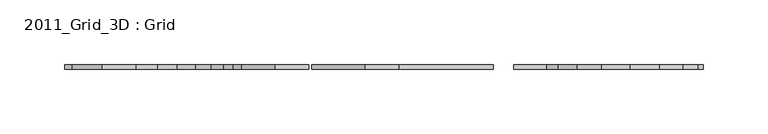
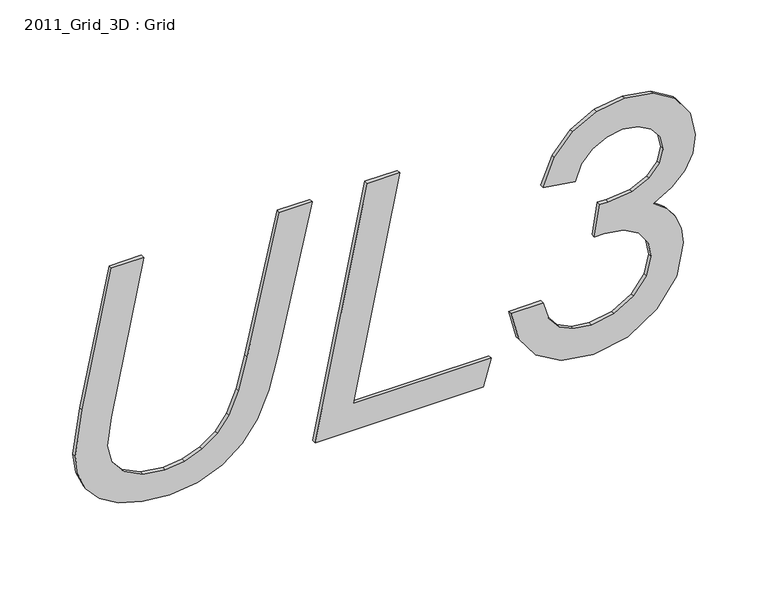
"""IFC4 building model written with IfcOpenShell, lengths in millimetres: proxy geometry, 2011_Grid_3D : Grid."""

from ifc_helpers import new_model, si_unit, frame, origin, place, context, project, spatial, polyline, outline, extrude, source, transform, mapped, element, save


def proxy_2011_grid_3d_grid_6e83494d(model_context):
    return source(origin(), model_context, "Body", "SweptSolid", [
        extrude(outline(polyline([(101.4447294, 32343.9093434), (-9.5457855, 32320.8090397), (-46.3278141, 32315.1578924), (-62.2836301, 32317.3018584), (-76.4424804, 32323.7337562), (-88.2714718, 32334.4659789), (-97.2377109, 32349.5109192), (-102.8888581, 32368.2985052), (-104.7725739, 32390.2586651), (-102.1081075, 32412.4542896), (-94.1147085, 32431.7499831), (-81.7032524, 32447.6500312), (-65.784615, 32459.6587191), (-44.9584024, 32468.7550833), (-17.8242205, 32475.9181603), (101.4447294, 32503.0833243), (101.4447294, 32477.157447), (-10.7355007, 32451.57857), (-36.7791103, 32444.8864219), (-54.6310349, 32437.4011304), (-66.7202764, 32428.1064803), (-75.4758368, 32415.9862566), (-80.7923767, 32401.9079599), (-82.5645566, 32386.739091), (-80.0983761, 32368.639309), (-72.6998347, 32353.897994), (-61.2488258, 32344.1014328), (-46.6252429, 32340.8359124), (-23.5745107, 32343.9589148), (101.4447294, 32369.6369348), (101.4447294, 32343.9093434)])), frame((0.0, -3.175, 0.0), z_axis=(0.0, 1.0, 0.0), x_axis=(0.0, 0.0, 1.0)), (0.0, 0.0, 1.0), 3.175),
        extrude(outline(polyline([(-101.6, 32505.5123262), (-101.6, 32638.7604299), (-79.3919827, 32645.1055777), (-79.3919827, 32535.8004926), (101.4447294, 32572.5329498), (101.4447294, 32546.7557869), (-101.6, 32505.5123262)])), frame((0.0, -3.175, 0.0), z_axis=(0.0, 1.0, 0.0), x_axis=(0.0, 0.0, 1.0)), (0.0, 0.0, 1.0), 3.175),
        extrude(outline(polyline([(-47.6662438, 32660.9684472), (-71.0391905, 32666.8178803), (-89.2071332, 32680.4004623), (-100.8812137, 32700.5760494), (-104.7725739, 32726.2044979), (-99.641927, 32753.3510726), (-84.2499865, 32776.3956084), (-61.8684691, 32792.1407456), (-35.7690916, 32797.3891247), (-23.320457, 32795.9267664), (-12.3465734, 32791.5396916), (-2.8598339, 32784.1783287), (5.1273687, 32773.7931064), (13.6970361, 32788.3733141), (24.2371693, 32798.7027686), (36.7477683, 32804.8558269), (51.2288332, 32806.9068464), (70.7352055, 32803.0340755), (86.9202895, 32791.4157629), (97.8136194, 32773.5514455), (101.4447294, 32750.94066), (98.0428874, 32728.7884106), (87.8373617, 32709.821128), (71.4106167, 32695.265706), (49.3451174, 32686.3490383), (45.2306856, 32711.7296295), (58.2865708, 32716.6495976), (68.0087748, 32725.361783), (74.0502974, 32736.6268989), (76.0641382, 32749.2056587), (74.0936724, 32761.734847), (68.1822749, 32772.1572479), (59.3833395, 32779.1840034), (48.7502598, 32781.5262552), (37.1877151, 32778.7688424), (27.5832433, 32770.4966038), (21.1141669, 32756.8830396), (18.9578081, 32738.10165), (19.4039513, 32731.2112161), (-6.4227831, 32726.9480699), (-6.4227831, 32734.9290761), (-8.6968742, 32750.1599094), (-15.5191473, 32761.9455257), (-25.8362089, 32769.4927816), (-38.5946653, 32772.0085335), (-53.7015699, 32768.5137451), (-66.9991159, 32758.0293798), (-76.293766, 32742.7365822), (-79.3919827, 32724.8164968), (-77.551642, 32710.3911999), (-72.0306199, 32699.0393339), (-62.2588444, 32690.9591848), (-47.6662438, 32686.3490383), (-47.6662438, 32660.9684472)])), frame((0.0, -3.175, 0.0), z_axis=(0.0, 1.0, 0.0), x_axis=(0.0, 0.0, 1.0)), (0.0, 0.0, 1.0), 3.175),
    ])


if __name__ == "__main__":
    model = new_model("IFC4")
    model_context = context("Model", 3, world=origin())
    ifc_project = project(units=[si_unit("LENGTHUNIT", "METRE", prefix="MILLI")], contexts=[model_context])
    site = spatial("IfcSite", under=ifc_project)
    building = spatial("IfcBuilding", under=site)
    placement = place(None, origin())
    proxy_2011_grid_3d_grid_shape = proxy_2011_grid_3d_grid_6e83494d(model_context)
    element("IfcBuildingElementProxy", 1, Name="2011_Grid_3D : Grid", ObjectType="2011_Grid_3D : Grid", at=placement, inside=building, context=model_context, shape_type="MappedRepresentation", body=[
        mapped(proxy_2011_grid_3d_grid_shape, transform((0.0, 0.0, 0.0), x_axis=(1.0, 0.0, 0.0), y_axis=(0.0, 1.0, 0.0), z_axis=(0.0, 0.0, 1.0))),
    ])
    save(model, "model.ifc")

# Revit data of these elements
# Type "2011_Grid_3D : Grid"
#   Workplane [instance default] = "LEVEL"
#   Grid [instance default] = "S"
#   t [instance default] = 12' - 6"
#   built-in parameter 1001306 [instance default] = 50 (stored number, unit not read)
#   d [instance default] = 2
#   Symbol At End 2 [instance default] = yes
#   Symbol At End 1 [instance default] = yes
#   Robust [instance default] = yes
#   No of grid markers [instance default] = 3
#   Grid Height Visible = yes
#   Height = 0
#   Assembly Code = ""
# Element 1 (IfcBuildingElementProxy, "2011_Grid_3D : Grid")
#   Workplane = "UL3"
#   Grid = "1"
#   t = 13' - 2.15638"
#   built-in parameter 1001306 = 105.438 (stored number, unit not read)
#   d = 4
#   Robust = no
#   No of grid markers = 5
#   Materials on its faces: "Letter"
# Materials
#   "Letter": class "Unassigned", colour RGB 178 187 30, transparency 0, Comments = "Rendering appearance not upgraded "
